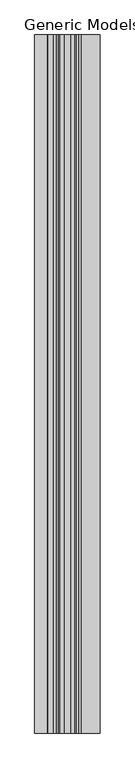
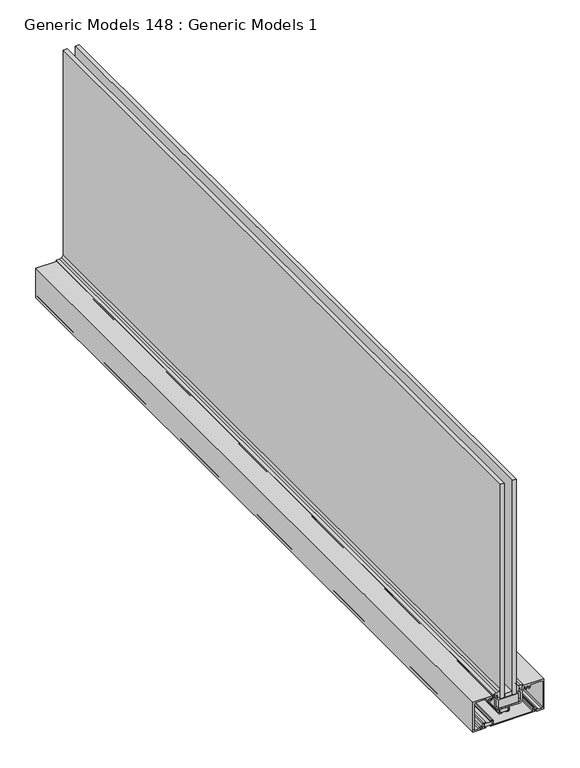
"""IFC4 building model written with IfcOpenShell, lengths in millimetres: proxy geometry, Generic Models 148 : Generic Models 1."""

from ifc_helpers import new_model, si_unit, point, frame, frame_2d, origin, place, context, project, spatial, polyline, circle_curve, trimmed, segment, composite_curve, outline, extrude, source, transform, mapped, element, save


def generic_models_148_generic_models_1_015d61f0(model_context):
    return source(origin(), model_context, "Body", "SweptSolid", [
        extrude(outline(composite_curve([segment(trimmed(circle_curve(frame_2d((14.097, 50917.5916343)), 1.5795625), [point((15.6765625, 50917.5916343))], [point((14.6380548, 50916.1076271))], False, "CARTESIAN"), True, "CONTINUOUS"), segment(polyline([(14.6380548, 50916.1076271), (10.7648375, 50914.6954892), (10.7648375, 50916.1851634), (8.1835625, 50916.1851634), (8.1835625, 50911.8671634), (6.5484375, 50911.8671634), (6.5484375, 50921.1478154), (8.1835625, 50921.1478154), (8.1835625, 50917.5664154), (14.8034375, 50917.5664154), (14.8034375, 50921.1478154), (15.6765625, 50921.1478154), (15.6765625, 50917.5916343)]), True, "CONTINUOUS")], self_intersect=False)), frame((0.0, 0.0, 0.0), z_axis=(0.0, 1.0, 0.0), x_axis=(0.0, 0.0, 1.0)), (0.0, 0.0, 1.0), 1219.2),
        extrude(outline(composite_curve([segment(trimmed(circle_curve(frame_2d((12.446, 50996.7010997)), 0.7064375), [point((12.6878975, 50997.3648312))], [point((11.740864, 50996.6582372))], True, "CARTESIAN"), True, "CONTINUOUS"), segment(polyline([(11.740864, 50996.6582372), (8.1835625, 50996.6582372), (8.1835625, 50933.5636529)]), True, "CONTINUOUS"), segment(trimmed(circle_curve(frame_2d((8.89, 50933.5636529)), 0.7064375), [point((8.1835625, 50933.5636529))], [point((8.89, 50932.8572154))], True, "CARTESIAN"), True, "CONTINUOUS"), segment(polyline([(8.89, 50932.8572154), (14.097, 50932.8572154)]), True, "CONTINUOUS"), segment(trimmed(circle_curve(frame_2d((14.097, 50931.2776529)), 1.5795625), [point((14.097, 50932.8572154))], [point((15.6765625, 50931.2776529))], False, "CARTESIAN"), True, "CONTINUOUS"), segment(polyline([(15.6765625, 50931.2776529), (15.6765625, 50927.8946904), (14.8034375, 50927.8946904), (14.8034375, 50931.4760904), (8.1835625, 50931.4760904), (8.1835625, 50927.8946904), (6.5484375, 50927.8946904), (6.5484375, 51002.3573622), (8.1835625, 51002.3573622), (8.1835625, 50998.0393622), (10.7648375, 50998.0393622), (10.7648375, 50999.5290364), (16.009985, 50997.616706)]), True, "CONTINUOUS"), segment(trimmed(circle_curve(frame_2d((15.7734, 50996.9677997)), 0.6906895), [point((16.009985, 50997.616706))], [point((15.5374141, 50996.3186752))], False, "CARTESIAN"), True, "CONTINUOUS"), segment(polyline([(15.5374141, 50996.3186752), (12.6878975, 50997.3648312)]), True, "CONTINUOUS")], self_intersect=False)), frame((0.0, 0.0, 0.0), z_axis=(0.0, 1.0, 0.0), x_axis=(0.0, 0.0, 1.0)), (0.0, 0.0, 1.0), 1219.2),
        extrude(outline(composite_curve([segment(trimmed(circle_curve(frame_2d((34.29, 50974.625)), 2.54), [point((34.29, 50977.165))], [point((31.75, 50974.625))], True, "CARTESIAN"), True, "CONTINUOUS"), segment(polyline([(31.75, 50974.625), (31.75, 50953.1493), (29.718, 50953.1493), (29.718, 50956.7307), (23.495, 50956.7307), (23.495, 50953.1493), (22.225, 50953.1493), (22.225, 50956.7307)]), True, "CONTINUOUS"), segment(trimmed(circle_curve(frame_2d((24.003, 50956.7307)), 1.778), [point((22.225, 50956.7307))], [point((24.003, 50958.5087))], False, "CARTESIAN"), True, "CONTINUOUS"), segment(polyline([(24.003, 50958.5087), (29.21, 50958.5087)]), True, "CONTINUOUS"), segment(trimmed(circle_curve(frame_2d((29.21, 50959.0167)), 0.508), [point((29.21, 50958.5087))], [point((29.718, 50959.0167))], True, "CARTESIAN"), True, "CONTINUOUS"), segment(polyline([(29.718, 50959.0167), (29.718, 50974.879)]), True, "CONTINUOUS"), segment(trimmed(circle_curve(frame_2d((34.036, 50974.879)), 4.318), [point((29.718, 50974.879))], [point((34.036, 50979.197))], False, "CARTESIAN"), True, "CONTINUOUS"), segment(polyline([(34.036, 50979.197), (49.1342256, 50979.197), (50.8386835, 50980.9028737)]), True, "CONTINUOUS"), segment(trimmed(circle_curve(frame_2d((52.7253201, 50979.017803)), 2.667), [point((50.8386835, 50980.9028737))], [point((52.7253201, 50981.684803))], False, "CARTESIAN"), True, "CONTINUOUS"), segment(polyline([(52.7253201, 50981.684803), (54.61, 50981.684803)]), True, "CONTINUOUS"), segment(trimmed(circle_curve(frame_2d((54.61, 50982.192803)), 0.508), [point((54.61, 50981.684803))], [point((55.118, 50982.192803))], True, "CARTESIAN"), True, "CONTINUOUS"), segment(polyline([(55.118, 50982.192803), (55.118, 50984.0043351)]), True, "CONTINUOUS"), segment(trimmed(circle_curve(frame_2d((54.61, 50984.0043351)), 0.508), [point((55.118, 50984.0043351))], [point((54.3683568, 50984.4511825))], True, "CARTESIAN"), True, "CONTINUOUS"), segment(trimmed(circle_curve(frame_2d((52.3748, 50988.137673)), 4.191), [point((54.3683568, 50984.4511825))], [point((49.3268, 50985.2611861))], False, "CARTESIAN"), True, "CONTINUOUS"), segment(polyline([(49.3268, 50985.2611861), (49.3268, 50986.3779094), (50.2850807, 50986.931173)]), True, "CONTINUOUS"), segment(trimmed(circle_curve(frame_2d((52.3748, 50988.137673)), 2.413), [point((50.2850807, 50986.931173))], [point((50.2850807, 50989.344173))], True, "CARTESIAN"), True, "CONTINUOUS"), segment(polyline([(50.2850807, 50989.344173), (49.3268, 50989.8974366), (49.3268, 50991.0141599)]), True, "CONTINUOUS"), segment(trimmed(circle_curve(frame_2d((52.3748, 50988.137673)), 4.191), [point((49.3268, 50991.0141599))], [point((54.3683568, 50991.8241635))], False, "CARTESIAN"), True, "CONTINUOUS"), segment(trimmed(circle_curve(frame_2d((54.61, 50992.2710109)), 0.508), [point((54.3683568, 50991.8241635))], [point((55.118, 50992.2710109))], True, "CARTESIAN"), True, "CONTINUOUS"), segment(polyline([(55.118, 50992.2710109), (55.118, 51010.756373)]), True, "CONTINUOUS"), segment(trimmed(circle_curve(frame_2d((53.594, 51010.756373)), 1.524), [point((55.118, 51010.756373))], [point((53.594, 51012.280373))], True, "CARTESIAN"), True, "CONTINUOUS"), segment(polyline([(53.594, 51012.280373), (9.906, 51012.280373)]), True, "CONTINUOUS"), segment(trimmed(circle_curve(frame_2d((9.906, 51010.756373)), 1.524), [point((9.906, 51012.280373))], [point((8.382, 51010.756373))], True, "CARTESIAN"), True, "CONTINUOUS"), segment(polyline([(8.382, 51010.756373), (8.382, 51004.700214)]), True, "CONTINUOUS"), segment(trimmed(circle_curve(frame_2d((8.89, 51003.263373)), 1.524), [point((8.382, 51004.700214))], [point((10.414, 51003.263373))], False, "CARTESIAN"), True, "CONTINUOUS"), segment(polyline([(10.414, 51003.263373), (10.414, 50998.5052015)]), True, "CONTINUOUS"), segment(trimmed(circle_curve(frame_2d((9.9568, 51000.012173)), 1.5748), [point((10.414, 50998.5052015))], [point((8.382, 51000.012173))], False, "CARTESIAN"), True, "CONTINUOUS"), segment(polyline([(8.382, 51000.012173), (8.382, 51002.755373), (6.35, 51002.755373), (6.35, 51014.312373), (57.15, 51014.312373), (57.15, 50979.652803), (52.46214, 50979.652803), (50.5841, 50977.773203), (50.5841, 50976.2991491), (53.5813, 50975.640873), (55.3593, 50975.640873), (55.3593, 50974.624873), (49.3141, 50974.624873), (49.3141, 50976.657)]), True, "CONTINUOUS"), segment(trimmed(circle_curve(frame_2d((48.8061, 50976.657)), 0.508), [point((49.3141, 50976.657))], [point((48.8061, 50977.165))], True, "CARTESIAN"), True, "CONTINUOUS"), segment(polyline([(48.8061, 50977.165), (34.29, 50977.165)]), True, "CONTINUOUS")], self_intersect=False)), frame((0.0, 0.0, 0.0), z_axis=(0.0, 1.0, 0.0), x_axis=(0.0, 0.0, 1.0)), (0.0, 0.0, 1.0), 1219.2),
        extrude(outline(composite_curve([segment(trimmed(circle_curve(frame_2d((48.8061, 50937.667873)), 0.508), [point((48.8061, 50937.159873))], [point((49.3141, 50937.667873))], True, "CARTESIAN"), True, "CONTINUOUS"), segment(polyline([(49.3141, 50937.667873), (49.3141, 50939.7), (55.3593, 50939.7), (55.3593, 50938.684), (53.5813, 50938.684), (50.5841, 50938.0257239), (50.5841, 50936.55167), (52.46214, 50934.67207), (57.15, 50934.67207), (57.15, 50900.0125), (6.35, 50900.0125), (6.35, 50911.5695), (8.382, 50911.5695), (8.382, 50914.3127)]), True, "CONTINUOUS"), segment(trimmed(circle_curve(frame_2d((9.9568, 50914.3127)), 1.5748), [point((8.382, 50914.3127))], [point((10.414, 50915.8196715))], False, "CARTESIAN"), True, "CONTINUOUS"), segment(polyline([(10.414, 50915.8196715), (10.414, 50911.0615)]), True, "CONTINUOUS"), segment(trimmed(circle_curve(frame_2d((8.89, 50911.0615)), 1.524), [point((10.414, 50911.0615))], [point((8.382, 50909.624659))], False, "CARTESIAN"), True, "CONTINUOUS"), segment(polyline([(8.382, 50909.624659), (8.382, 50903.568373)]), True, "CONTINUOUS"), segment(trimmed(circle_curve(frame_2d((9.906, 50903.568373)), 1.524), [point((8.382, 50903.568373))], [point((9.906, 50902.044373))], True, "CARTESIAN"), True, "CONTINUOUS"), segment(polyline([(9.906, 50902.044373), (53.594, 50902.044373)]), True, "CONTINUOUS"), segment(trimmed(circle_curve(frame_2d((53.594, 50903.568373)), 1.524), [point((53.594, 50902.044373))], [point((55.118, 50903.568373))], True, "CARTESIAN"), True, "CONTINUOUS"), segment(polyline([(55.118, 50903.568373), (55.118, 50922.0538621)]), True, "CONTINUOUS"), segment(trimmed(circle_curve(frame_2d((54.61, 50922.0538621)), 0.508), [point((55.118, 50922.0538621))], [point((54.3683568, 50922.5007095))], True, "CARTESIAN"), True, "CONTINUOUS"), segment(trimmed(circle_curve(frame_2d((52.3748, 50926.1872)), 4.191), [point((54.3683568, 50922.5007095))], [point((49.3268, 50923.3107131))], False, "CARTESIAN"), True, "CONTINUOUS"), segment(polyline([(49.3268, 50923.3107131), (49.3268, 50924.4274364), (50.2850807, 50924.9807)]), True, "CONTINUOUS"), segment(trimmed(circle_curve(frame_2d((52.3748, 50926.1872)), 2.413), [point((50.2850807, 50924.9807))], [point((50.2850807, 50927.3937))], True, "CARTESIAN"), True, "CONTINUOUS"), segment(polyline([(50.2850807, 50927.3937), (49.3268, 50927.9469636), (49.3268, 50929.0636869)]), True, "CONTINUOUS"), segment(trimmed(circle_curve(frame_2d((52.3748, 50926.1872)), 4.191), [point((49.3268, 50929.0636869))], [point((54.3683568, 50929.8736905))], False, "CARTESIAN"), True, "CONTINUOUS"), segment(trimmed(circle_curve(frame_2d((54.61, 50930.3205379)), 0.508), [point((54.3683568, 50929.8736905))], [point((55.118, 50930.3205379))], True, "CARTESIAN"), True, "CONTINUOUS"), segment(polyline([(55.118, 50930.3205379), (55.118, 50932.13207)]), True, "CONTINUOUS"), segment(trimmed(circle_curve(frame_2d((54.61, 50932.13207)), 0.508), [point((55.118, 50932.13207))], [point((54.61, 50932.64007))], True, "CARTESIAN"), True, "CONTINUOUS"), segment(polyline([(54.61, 50932.64007), (52.7253201, 50932.64007)]), True, "CONTINUOUS"), segment(trimmed(circle_curve(frame_2d((52.7253201, 50935.30707)), 2.667), [point((52.7253201, 50932.64007))], [point((50.8386835, 50933.4219993))], False, "CARTESIAN"), True, "CONTINUOUS"), segment(polyline([(50.8386835, 50933.4219993), (49.1342256, 50935.127873), (34.036, 50935.127873)]), True, "CONTINUOUS"), segment(trimmed(circle_curve(frame_2d((34.036, 50939.445873)), 4.318), [point((34.036, 50935.127873))], [point((29.718, 50939.445873))], False, "CARTESIAN"), True, "CONTINUOUS"), segment(polyline([(29.718, 50939.445873), (29.718, 50941.439773), (24.003, 50941.439773)]), True, "CONTINUOUS"), segment(trimmed(circle_curve(frame_2d((24.003, 50943.217773)), 1.778), [point((24.003, 50941.439773))], [point((22.225, 50943.217773))], False, "CARTESIAN"), True, "CONTINUOUS"), segment(polyline([(22.225, 50943.217773), (22.225, 50946.7993), (23.495, 50946.7993), (23.495, 50943.2179), (29.718, 50943.2179), (29.718, 50946.7993), (31.75, 50946.7993), (31.75, 50939.699873)]), True, "CONTINUOUS"), segment(trimmed(circle_curve(frame_2d((34.29, 50939.699873)), 2.54), [point((31.75, 50939.699873))], [point((34.29, 50937.159873))], True, "CARTESIAN"), True, "CONTINUOUS"), segment(polyline([(34.29, 50937.159873), (48.8061, 50937.159873)]), True, "CONTINUOUS")], self_intersect=False)), frame((0.0, 0.0, 0.0), z_axis=(0.0, 1.0, 0.0), x_axis=(0.0, 0.0, 1.0)), (0.0, 0.0, 1.0), 1219.2),
        extrude(outline(polyline([(50973.0629678, 0.0), (50941.7098428, 0.0), (50941.7098428, 1219.2), (50973.0629678, 1219.2), (50973.0629678, 0.0)])), frame((0.0, 0.0, 32.5992301), z_axis=(0.0, 0.0, 1.0), x_axis=(1.0, 0.0, 0.0)), (0.0, 0.0, 1.0), 14.684375),
        extrude(outline(polyline([(50950.82359, 0.0), (50944.47359, 0.0), (50944.47359, 1219.2), (50950.82359, 1219.2), (50950.82359, 0.0)])), frame((0.0, 0.0, 47.625), z_axis=(0.0, 0.0, 1.0), x_axis=(1.0, 0.0, 0.0)), (0.0, 0.0, 1.0), 365.125),
        extrude(outline(polyline([(50969.87359, 0.0), (50963.52359, 0.0), (50963.52359, 1219.2), (50969.87359, 1219.2), (50969.87359, 0.0)])), frame((0.0, 0.0, 47.625), z_axis=(0.0, 0.0, 1.0), x_axis=(1.0, 0.0, 0.0)), (0.0, 0.0, 1.0), 365.125),
        extrude(outline(polyline([(50963.3251525, 0.0), (50951.0220275, 0.0), (50951.0220275, 1219.2), (50963.3251525, 1219.2), (50963.3251525, 0.0)])), frame((0.0, 0.0, 47.625), z_axis=(0.0, 0.0, 1.0), x_axis=(1.0, 0.0, 0.0)), (0.0, 0.0, 1.0), 6.35),
        extrude(outline(composite_curve([segment(trimmed(circle_curve(frame_2d((64.2304882, 50976.1426745)), 4.9643345), [point((59.3077698, 50976.7841265))], [point((60.6315489, 50972.7232808))], True, "CARTESIAN"), True, "CONTINUOUS"), segment(polyline([(60.6315489, 50972.7232808), (63.5908154, 50970.1744071), (50.679329, 50970.1744071), (50.679329, 50974.1558571), (56.1304866, 50974.1558571), (56.1304866, 50975.8945302), (54.2354153, 50975.8945302), (51.2348926, 50976.553536), (51.2348926, 50977.5441268), (52.8805452, 50979.1911463), (57.5342084, 50979.1911463), (57.5342084, 50980.9684916), (58.6865882, 50980.9684916)]), True, "CONTINUOUS"), segment(trimmed(circle_curve(frame_2d((47.3152777, 50977.1420956)), 11.9978335), [point((58.6865882, 50980.9684916))], [point((59.3077698, 50976.7841265))], False, "CARTESIAN"), True, "CONTINUOUS")], self_intersect=False)), frame((0.0, 0.0, 0.0), z_axis=(0.0, 1.0, 0.0), x_axis=(0.0, 0.0, 1.0)), (0.0, 0.0, 1.0), 1219.2),
        extrude(outline(composite_curve([segment(trimmed(circle_curve(frame_2d((47.3152777, 50937.0578364)), 11.9978335), [point((59.3077698, 50937.4158055))], [point((58.6865882, 50933.2314404))], False, "CARTESIAN"), True, "CONTINUOUS"), segment(polyline([(58.6865882, 50933.2314404), (57.5342084, 50933.2314404), (57.5342084, 50935.0087857), (52.8805452, 50935.0087857), (51.2348926, 50936.6558052), (51.2348926, 50937.646396), (54.2354153, 50938.3054018), (56.1304866, 50938.3054018), (56.1304866, 50940.0440749), (50.679329, 50940.0440749), (50.679329, 50944.0255249), (63.5908154, 50944.0255249), (60.6315489, 50941.4766512)]), True, "CONTINUOUS"), segment(trimmed(circle_curve(frame_2d((64.2304882, 50938.0572575)), 4.9643345), [point((60.6315489, 50941.4766512))], [point((59.3077698, 50937.4158055))], True, "CARTESIAN"), True, "CONTINUOUS")], self_intersect=False)), frame((0.0, 0.0, 0.0), z_axis=(0.0, 1.0, 0.0), x_axis=(0.0, 0.0, 1.0)), (0.0, 0.0, 1.0), 1219.2),
        extrude(outline(polyline([(50931.0792154, 0.0), (50917.9632904, 0.0), (50917.9632904, 1219.2), (50931.0792154, 1219.2), (50931.0792154, 0.0)])), frame((0.0, 0.0, 8.5804375), z_axis=(0.0, 0.0, 1.0), x_axis=(1.0, 0.0, 0.0)), (0.0, 0.0, 1.0), 5.826125),
        extrude(outline(polyline([(50956.5322625, 0.0), (50943.4163375, 0.0), (50943.4163375, 1219.2), (50956.5322625, 1219.2), (50956.5322625, 0.0)])), frame((0.0, 0.0, 23.6934375), z_axis=(0.0, 0.0, 1.0), x_axis=(1.0, 0.0, 0.0)), (0.0, 0.0, 1.0), 5.826125),
    ])


if __name__ == "__main__":
    model = new_model("IFC4")
    model_context = context("Model", 3, world=origin())
    ifc_project = project(units=[si_unit("LENGTHUNIT", "METRE", prefix="MILLI")], contexts=[model_context])
    site = spatial("IfcSite", under=ifc_project)
    building = spatial("IfcBuilding", under=site)
    placement = place(None, origin())
    generic_models_148_generic_models_1_shape = generic_models_148_generic_models_1_015d61f0(model_context)
    element("IfcBuildingElementProxy", 1, Name="Generic Models 148 : Generic Models 1", ObjectType="Generic Models 148 : Generic Models 1", at=placement, inside=building, context=model_context, shape_type="MappedRepresentation", body=[
        mapped(generic_models_148_generic_models_1_shape, transform((0.0, 0.0, 0.0), x_axis=(1.0, 0.0, 0.0), y_axis=(0.0, 1.0, 0.0), z_axis=(0.0, 0.0, 1.0))),
    ])
    save(model, "model.ifc")

# Revit data of these elements
# Project information
#   Project Issue Date = "05/20/2019"
#   Project Status = "Project Status"
#   Client Name = "Owner"
#   Project Address = "SOMERS, WI"
#   Project Name = "OAKFIRE 2.0"
#   Project Number = "Project Number"
# Element 1 (IfcBuildingElementProxy, "Generic Models 148 : Generic Models 1")
#   Materials on its faces: "ALUM. STOREFRONT W/ INSULATED GLAZING"
# Materials
#   "ALUM. STOREFRONT W/ INSULATED GLAZING": class "Glass", colour RGB 196 205 210, transparency 0.85, Description = "Soda Lime Glass", Cost = 0
